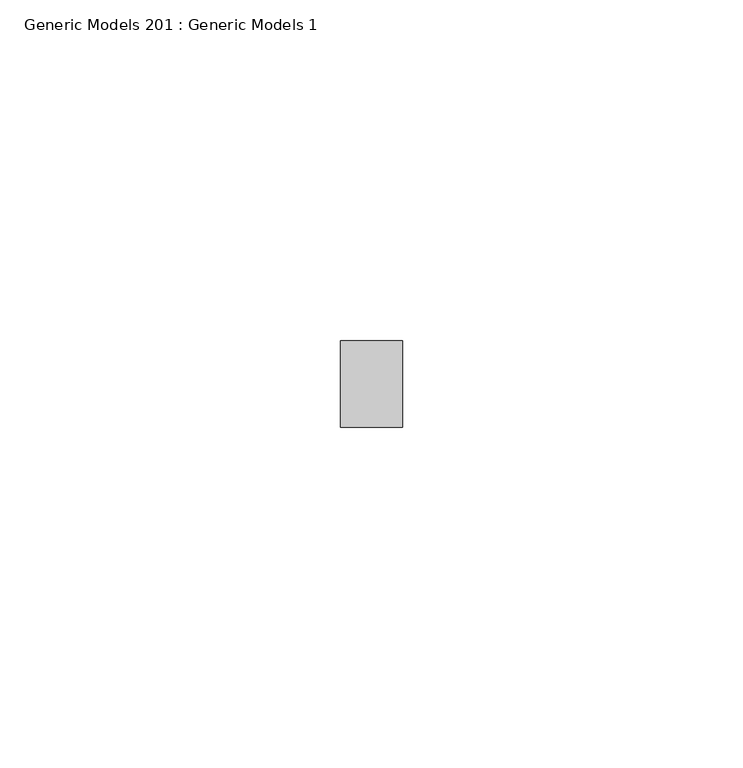
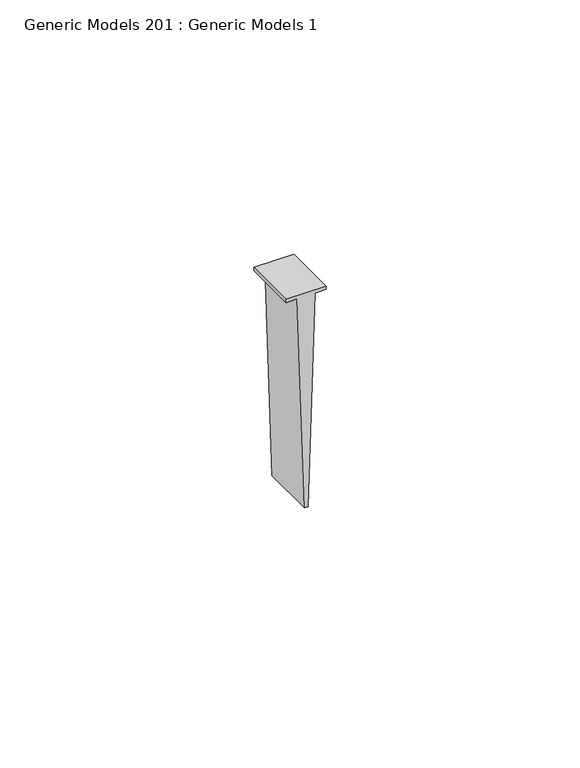
"""IFC4 building model written with IfcOpenShell, lengths in millimetres: proxy geometry, Generic Models 201 : Generic Models 1."""

import ifcopenshell
import ifcopenshell.guid

model = None  # the IFC model being written
_history = None  # IfcOwnerHistory: only IFC2X3 demands one
_inside = {}  # id of a spatial element -> (the spatial element, [elements in it])
_under = {}  # id of a project, library or spatial element -> (it, [spatial elements below it])
_declared = {}  # id of a project -> (the project, [libraries it declares])
_typed = {}  # id of a type object -> (the type object, [elements of that type])
_made_of = {}  # id of a material, layer set ... -> (it, [elements and type objects made of it])


def new_model(schema):
    """Start an empty IFC model of exactly this schema.

    Asked for "IFC4X3", IfcOpenShell would pick the latest addendum, in which some entities
    have other attributes; the version numbers below select the first issue.
    IFC2X3 requires an IfcOwnerHistory on every rooted entity: one is made here for all.
    """
    global model, _history
    if schema == "IFC4X3":
        model = ifcopenshell.file(schema_version=(4, 3, 0, 0))
    else:
        model = ifcopenshell.file(schema=schema)
    _inside.clear()
    _under.clear()
    _declared.clear()
    _typed.clear()
    _made_of.clear()
    _history = None
    if model.schema == "IFC2X3":
        org = make("IfcOrganization", Name="unknown")
        user = make(
            "IfcPersonAndOrganization",
            ThePerson=make("IfcPerson", FamilyName="unknown"),
            TheOrganization=org,
        )
        app = make(
            "IfcApplication",
            ApplicationDeveloper=org,
            Version="unknown",
            ApplicationFullName="unknown",
            ApplicationIdentifier="unknown",
        )
        _history = make(
            "IfcOwnerHistory",
            OwningUser=user,
            OwningApplication=app,
            ChangeAction="ADDED",
            CreationDate=0,
        )
    return model


def make(cls, **values):
    """One entity of the class cls with the attributes given. An attribute that is None is left unset."""
    return model.create_entity(
        cls, **{name: value for name, value in values.items() if value is not None}
    )


def rooted(cls, **values):
    """An entity with a GlobalId (a new one), such as an element, a storey or a relation."""
    return make(cls, GlobalId=ifcopenshell.guid.new(), OwnerHistory=_history, **values)


def si_unit(unit_type, name, prefix=None):
    """IfcSIUnit, for example si_unit("LENGTHUNIT", "METRE", prefix="MILLI")."""
    return make("IfcSIUnit", UnitType=unit_type, Prefix=prefix, Name=name)


def assignment(units):
    """IfcUnitAssignment: the units of a project."""
    return None if units is None else make("IfcUnitAssignment", Units=units)


def point(xyz):
    """IfcCartesianPoint."""
    return None if xyz is None else make("IfcCartesianPoint", Coordinates=xyz)


def direction(xyz):
    """IfcDirection."""
    return None if xyz is None else make("IfcDirection", DirectionRatios=xyz)


def frame(location, z_axis=None, x_axis=None):
    """IfcAxis2Placement3D, a coordinate frame: its origin and axes. An axis left out is left unset."""
    return make(
        "IfcAxis2Placement3D",
        Location=point(location),
        Axis=direction(z_axis),
        RefDirection=direction(x_axis),
    )


def origin():
    """The frame at (0, 0, 0) with its axes left unset."""
    return frame((0.0, 0.0, 0.0))


def place(relative_to, where):
    """IfcLocalPlacement: puts the frame where relative to a parent placement (None: the world)."""
    return make(
        "IfcLocalPlacement", PlacementRelTo=relative_to, RelativePlacement=where
    )


def context(
    kind, dimensions, precision=None, world=None, true_north=None, identifier=None
):
    """IfcGeometricRepresentationContext, for example the 3D "Model" context."""
    return make(
        "IfcGeometricRepresentationContext",
        ContextIdentifier=identifier,
        ContextType=kind,
        CoordinateSpaceDimension=dimensions,
        Precision=precision,
        WorldCoordinateSystem=world,
        TrueNorth=true_north,
    )


def project(units=None, contexts=None):
    """IfcProject with its units and contexts."""
    return rooted(
        "IfcProject",
        Name="project",
        RepresentationContexts=contexts,
        UnitsInContext=assignment(units),
    )


def spatial(cls, under=None, at=None, **own):
    """A site, building, storey or space (cls), placed at a placement, below another one or the project."""
    s = rooted(cls, ObjectPlacement=at, **own)
    if under is not None:
        _under.setdefault(under.id(), (under, []))[1].append(s)
    return s


def polyline(points):
    """IfcPolyline through the points."""
    return make("IfcPolyline", Points=[point(p) for p in points])


def outline(outer, holes=None, kind="AREA"):
    """IfcArbitraryClosedProfileDef: a profile drawn as a closed curve; with holes, ...WithVoids."""
    if holes is None:
        return make("IfcArbitraryClosedProfileDef", ProfileType=kind, OuterCurve=outer)
    return make(
        "IfcArbitraryProfileDefWithVoids",
        ProfileType=kind,
        OuterCurve=outer,
        InnerCurves=holes,
    )


def extrude(swept, where, along, depth):
    """IfcExtrudedAreaSolid: the profile swept, set in the frame where, extruded along a direction by depth."""
    return make(
        "IfcExtrudedAreaSolid",
        SweptArea=swept,
        Position=where,
        ExtrudedDirection=direction(along),
        Depth=depth,
    )


def shape(context_of_items, identifier, shape_type, items):
    """IfcShapeRepresentation: the items that make up one representation, for example the "Body"."""
    return make(
        "IfcShapeRepresentation",
        ContextOfItems=context_of_items,
        RepresentationIdentifier=identifier,
        RepresentationType=shape_type,
        Items=items,
    )


def source(mapping_origin, context_of_items, identifier, shape_type, items):
    """IfcRepresentationMap: a shape defined once, which mapped items show again and again."""
    return make(
        "IfcRepresentationMap",
        MappingOrigin=mapping_origin,
        MappedRepresentation=shape(context_of_items, identifier, shape_type, items),
    )


def transform(
    local_origin,
    x_axis=None,
    y_axis=None,
    z_axis=None,
    scale=None,
    scale2=None,
    scale3=None,
    uniform=True,
):
    """IfcCartesianTransformationOperator3D, or its non-uniform kind. x_axis, y_axis, z_axis: its Axis1, 2, 3."""
    if uniform:
        return make(
            "IfcCartesianTransformationOperator3D",
            Axis1=direction(x_axis),
            Axis2=direction(y_axis),
            LocalOrigin=point(local_origin),
            Scale=scale,
            Axis3=direction(z_axis),
        )
    return make(
        "IfcCartesianTransformationOperator3DnonUniform",
        Axis1=direction(x_axis),
        Axis2=direction(y_axis),
        LocalOrigin=point(local_origin),
        Scale=scale,
        Axis3=direction(z_axis),
        Scale2=scale2,
        Scale3=scale3,
    )


def mapped(mapping_source, mapping_target):
    """IfcMappedItem: shows the shape of a source again, moved by a transform."""
    return make(
        "IfcMappedItem", MappingSource=mapping_source, MappingTarget=mapping_target
    )


def made_of(thing, what):
    """Note that an element or type object is made of a material, layer set ...; save() writes the relation."""
    if what is not None:
        _made_of.setdefault(what.id(), (what, []))[1].append(thing)
    return thing


def element(
    cls,
    number,
    at=None,
    inside=None,
    cuts=None,
    type_object=None,
    material=None,
    context=None,
    identifier="Body",
    shape_type=None,
    held_by="IfcProductDefinitionShape",
    body=None,
    shapes=None,
    **own,
):
    """One element of the class cls, such as IfcWall. Its Tag is "e" and its number.

    at: its placement. inside: the storey or other place that contains it. cuts: it is an
    opening in that element (IfcRelVoidsElement). A single representation is given by context,
    identifier, shape_type and body (its items); several are given by shapes. held_by: the class
    of the entity that holds the representations. save() writes the other relations.
    """
    e = rooted(cls, Tag="e%d" % number, ObjectPlacement=at, **own)
    if body is not None:
        shapes = [shape(context, identifier, shape_type, body)]
    if shapes is not None:
        e.Representation = make(held_by, Representations=shapes)
    if inside is not None:
        _inside.setdefault(inside.id(), (inside, []))[1].append(e)
    if cuts is not None:
        rooted(
            "IfcRelVoidsElement", RelatingBuildingElement=cuts, RelatedOpeningElement=e
        )
    if type_object is not None:
        _typed.setdefault(type_object.id(), (type_object, []))[1].append(e)
    return made_of(e, material)


def aggregate(whole, parts):
    """IfcRelAggregates: a whole, such as a stair, and the parts it consists of."""
    return rooted("IfcRelAggregates", RelatingObject=whole, RelatedObjects=parts)


def save(model, path):
    """Write the relations noted so far, then the file.

    IfcRelAggregates (storeys below a building ...), IfcRelContainedInSpatialStructure (elements
    in a storey), IfcRelDefinesByType, IfcRelAssociatesMaterial and IfcRelDeclares: one each for
    every whole, place, type object, material and project.
    """
    for whole, parts in _under.values():
        aggregate(whole, parts)
    for where, things in _inside.values():
        rooted(
            "IfcRelContainedInSpatialStructure",
            RelatedElements=things,
            RelatingStructure=where,
        )
    for kind, things in _typed.values():
        rooted("IfcRelDefinesByType", RelatedObjects=things, RelatingType=kind)
    for what, things in _made_of.values():
        rooted("IfcRelAssociatesMaterial", RelatedObjects=things, RelatingMaterial=what)
    for by, libraries in _declared.values():
        rooted("IfcRelDeclares", RelatingContext=by, RelatedDefinitions=libraries)
    model.write(path)


def generic_models_201_generic_models_1_6cd63f98(model_context):
    return source(origin(), model_context, "Body", "SweptSolid", [
        extrude(outline(polyline([(2.38125, 49733.4159), (1.5875, 49733.4159), (1.5875, 49735.9657636), (-49.2125, 49737.5631527), (-49.2125, 49738.3618473), (1.5875, 49739.9592364), (1.5875, 49742.5091), (2.38125, 49742.5091), (2.38125, 49733.4159)])), frame((0.0, 565.15, 0.0), z_axis=(0.0, 1.0, 0.0), x_axis=(0.0, 0.0, 1.0)), (0.0, 0.0, 1.0), 12.7),
    ])


if __name__ == "__main__":
    model = new_model("IFC4")
    model_context = context("Model", 3, world=origin())
    ifc_project = project(units=[si_unit("LENGTHUNIT", "METRE", prefix="MILLI")], contexts=[model_context])
    site = spatial("IfcSite", under=ifc_project)
    building = spatial("IfcBuilding", under=site)
    placement = place(None, origin())
    generic_models_201_generic_models_1_shape = generic_models_201_generic_models_1_6cd63f98(model_context)
    element("IfcBuildingElementProxy", 1, Name="Generic Models 201 : Generic Models 1", ObjectType="Generic Models 201 : Generic Models 1", at=placement, inside=building, context=model_context, shape_type="MappedRepresentation", body=[
        mapped(generic_models_201_generic_models_1_shape, transform((0.0, 0.0, 0.0), x_axis=(1.0, 0.0, 0.0), y_axis=(0.0, 1.0, 0.0), z_axis=(0.0, 0.0, 1.0))),
    ])
    save(model, "model.ifc")

# Revit data of these elements
# Element 1 (IfcBuildingElementProxy, "Generic Models 201 : Generic Models 1")
#   Materials on its faces: "METAL RUNNER CHANNEL; FASTEN @ 24\" O.C."
# Materials
#   "METAL RUNNER CHANNEL; FASTEN @ 24\" O.C.": class "Unassigned", colour RGB 210 209 208, transparency 0, Keynote = "M05121300.02", Cost = 0
